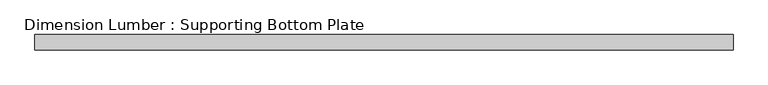
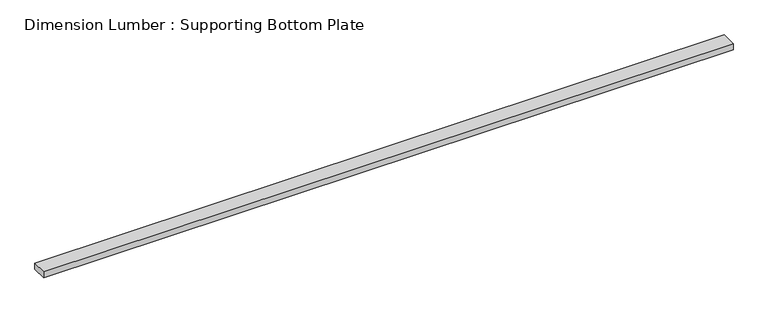
"""IFC4 building model written with IfcOpenShell, lengths in millimetres: beam geometry, Dimension Lumber : Supporting Bottom Plate."""

from ifc_helpers import new_model, si_unit, frame, origin, place, context, project, spatial, polyline, outline, extrude, source, transform, mapped, element, save


def dimension_lumber_supporting_bottom_plate_879a6a2b(model_context):
    return source(origin(), model_context, "Body", "SweptSolid", [
        extrude(outline(polyline([(2009.775, 44.45), (2009.775, -44.45), (-2060.575, -44.45), (-2060.575, 44.45), (2009.775, 44.45)])), frame((0.0, 0.0, -19.05), z_axis=(0.0, 0.0, 1.0), x_axis=(1.0, 0.0, 0.0)), (0.0, 0.0, 1.0), 38.1),
    ])


if __name__ == "__main__":
    model = new_model("IFC4")
    model_context = context("Model", 3, world=origin())
    ifc_project = project(units=[si_unit("LENGTHUNIT", "METRE", prefix="MILLI")], contexts=[model_context])
    site = spatial("IfcSite", under=ifc_project)
    building = spatial("IfcBuilding", under=site)
    placement = place(None, origin())
    dimension_lumber_supporting_bottom_plate_shape = dimension_lumber_supporting_bottom_plate_879a6a2b(model_context)
    element("IfcBeam", 1, ObjectType="Dimension Lumber : Supporting Bottom Plate", at=placement, inside=building, context=model_context, shape_type="MappedRepresentation", body=[
        mapped(dimension_lumber_supporting_bottom_plate_shape, transform((0.0, 0.0, 0.0), x_axis=(1.0, 0.0, 0.0), y_axis=(0.0, 1.0, 0.0), z_axis=(0.0, 0.0, 1.0))),
    ])
    save(model, "model.ifc")

# Revit data of these elements
# Type "Dimension Lumber : Supporting Bottom Plate"
#   Assembly Code = "B10"
#   A = 0.0364583 SF
#   Length [instance default] = 5' - 0"
#   b = 0' - 3 1/2"
#   d = 0' - 1 1/2"
#   Structural Material [instance default] = Softwood, Lumber
# Element 1 (IfcBeam, "Dimension Lumber : Supporting Bottom Plate")
#   Structural Material = Douglas Fir #2
#   Materials on its faces: "Douglas Fir #2"
# Materials
#   "Softwood, Lumber": class "Wood", colour RGB 223 192 134, transparency 0, Description = "Pinus Echinata", Cost = 0
#   "Douglas Fir #2": class "Wood", colour RGB 223 192 134, transparency 0, Description = "Pinus Echinata", Cost = 0
